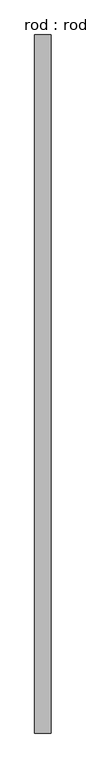
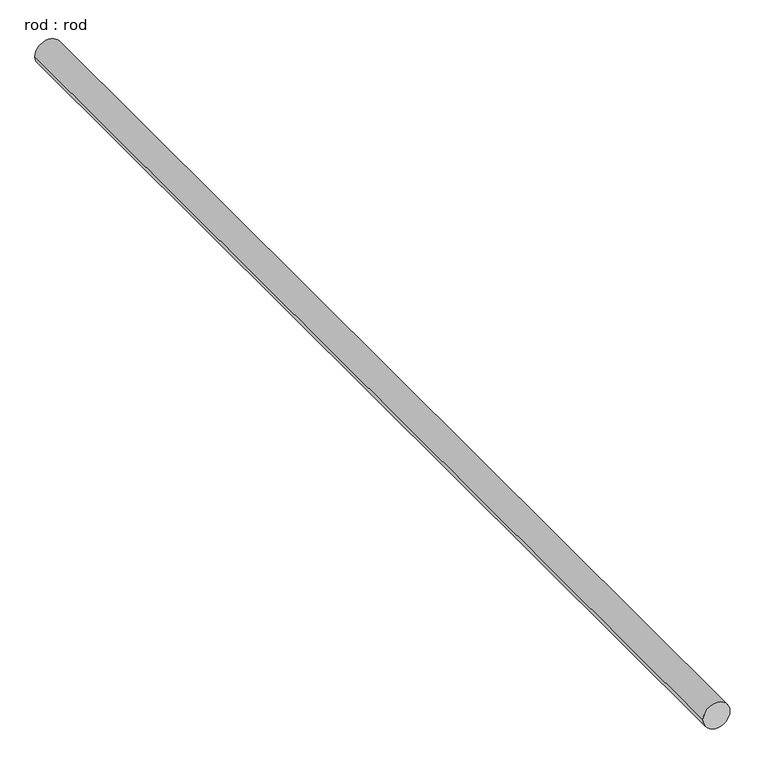
"""IFC4 building model written with IfcOpenShell, lengths in millimetres: proxy geometry, rod : rod."""

from ifc_helpers import new_model, si_unit, point, frame, frame_2d, origin, place, context, project, spatial, circle_curve, trimmed, segment, composite_curve, outline, extrude, source, transform, mapped, element, save


def rod_rod_0a9bb205(model_context):
    return source(origin(), model_context, "Body", "SweptSolid", [
        extrude(outline(composite_curve([segment(trimmed(circle_curve(frame_2d((0.0108462, 0.0)), 200.0), [point((0.0108462, 200.0))], [point((0.0108462, -200.0))], False, "CARTESIAN"), True, "CONTINUOUS"), segment(trimmed(circle_curve(frame_2d((0.0108462, 0.0)), 200.0), [point((0.0108462, -200.0))], [point((0.0108462, 200.0))], False, "CARTESIAN"), True, "CONTINUOUS")], self_intersect=False)), frame((0.0, -4482.6379117, 0.0), z_axis=(0.0, 1.0, 0.0), x_axis=(0.0, 0.0, 1.0)), (0.0, 0.0, 1.0), 17150.7330541),
    ])


if __name__ == "__main__":
    model = new_model("IFC4")
    model_context = context("Model", 3, world=origin())
    ifc_project = project(units=[si_unit("LENGTHUNIT", "METRE", prefix="MILLI")], contexts=[model_context])
    site = spatial("IfcSite", under=ifc_project)
    building = spatial("IfcBuilding", under=site)
    placement = place(None, origin())
    rod_rod_shape = rod_rod_0a9bb205(model_context)
    element("IfcBuildingElementProxy", 1, Name="rod : rod", ObjectType="rod : rod", at=placement, inside=building, context=model_context, shape_type="MappedRepresentation", body=[
        mapped(rod_rod_shape, transform((0.0, 0.0, 0.0), x_axis=(1.0, 0.0, 0.0), y_axis=(0.0, 1.0, 0.0), z_axis=(0.0, 0.0, 1.0))),
    ])
    save(model, "model.ifc")

# Revit data of these elements
# Type "rod : rod"
#   Default Elevation = 0
